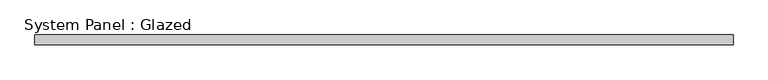
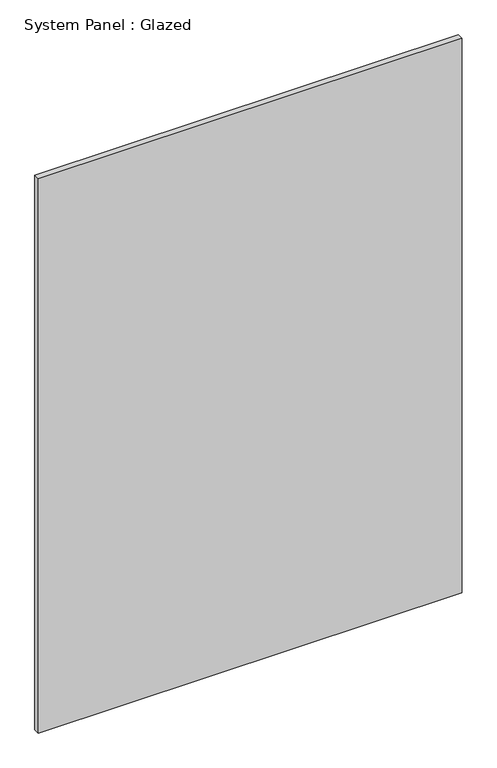
"""IFC4 building model written with IfcOpenShell, lengths in millimetres: plate geometry, System Panel : Glazed."""

from ifc_helpers import new_model, si_unit, origin, origin_with_axes, place, context, project, spatial, polyline, outline, extrude, source, transform, mapped, element, save


def system_panel_glazed_d09d15a5(model_context):
    return source(origin(), model_context, "Body", "SweptSolid", [
        extrude(outline(polyline([(877.5, -49.5), (-877.5, -49.5), (-877.5, -24.5), (877.5, -24.5), (877.5, -49.5)])), origin_with_axes(), (0.0, 0.0, 1.0), 2425.0),
    ])


if __name__ == "__main__":
    model = new_model("IFC4")
    model_context = context("Model", 3, world=origin())
    ifc_project = project(units=[si_unit("LENGTHUNIT", "METRE", prefix="MILLI")], contexts=[model_context])
    site = spatial("IfcSite", under=ifc_project)
    building = spatial("IfcBuilding", under=site)
    placement = place(None, origin())
    system_panel_glazed_shape = system_panel_glazed_d09d15a5(model_context)
    element("IfcPlate", 1, ObjectType="System Panel : Glazed", at=placement, inside=building, context=model_context, shape_type="MappedRepresentation", body=[
        mapped(system_panel_glazed_shape, transform((0.0, 0.0, 0.0), x_axis=(1.0, 0.0, 0.0), y_axis=(0.0, 1.0, 0.0), z_axis=(0.0, 0.0, 1.0))),
    ])
    save(model, "model.ifc")

# Revit data of these elements
# Type "System Panel : Glazed"
#   Keynote = "H11"
#   Construction Type Id = "GSP4R"
#   Analytic Construction = "1/8 in Pilkington single glazing"
#   Visual Light Transmittance = 0.9
#   Solar Heat Gain Coefficient = 0.86
#   Heat Transfer Coefficient (U) = 6.7069 W/(m²·K)
# Element 1 (IfcPlate, "System Panel : Glazed")
#   Materials on its faces: "Glass"
# Materials
#   "Glass": class "Glass", colour RGB 0 128 192, transparency 0.9, Description = "Soda Lime Glass", Cost = 0
